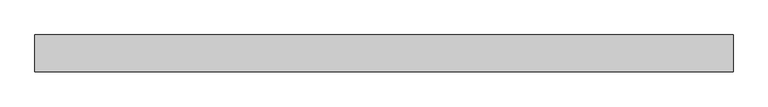
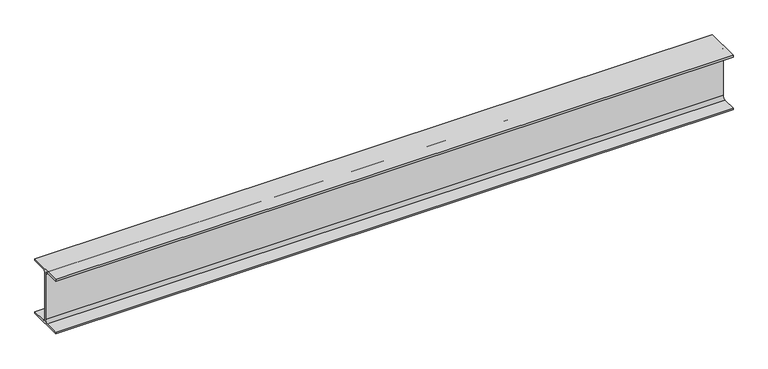
"""IFC4 building model written with IfcOpenShell, lengths in millimetres: beam geometry, 0912_Steel Framing_H-KSD3502 : H_SB_ASB_H-482x300x11x15."""

from ifc_helpers import new_model, si_unit, point, frame, frame_2d, origin, place, context, project, spatial, polyline, circle_curve, trimmed, segment, composite_curve, outline, extrude, source, transform, mapped, element, save


def beam_2ebcb970(model_context):
    return source(origin(), model_context, "Body", "SweptSolid", [
        extrude(outline(composite_curve([segment(polyline([(150.0, -226.0), (150.0, -241.0), (-150.0, -241.0), (-150.0, -226.0), (-31.5, -226.0)]), True, "CONTINUOUS"), segment(trimmed(circle_curve(frame_2d((-31.5, -200.0)), 26.0), [point((-31.5, -226.0))], [point((-5.5, -200.0))], True, "CARTESIAN"), True, "CONTINUOUS"), segment(polyline([(-5.5, -200.0), (-5.5, 200.0)]), True, "CONTINUOUS"), segment(trimmed(circle_curve(frame_2d((-31.5, 200.0)), 26.0), [point((-5.5, 200.0))], [point((-31.5, 226.0))], True, "CARTESIAN"), True, "CONTINUOUS"), segment(polyline([(-31.5, 226.0), (-150.0, 226.0), (-150.0, 241.0), (150.0, 241.0), (150.0, 226.0), (31.5, 226.0)]), True, "CONTINUOUS"), segment(trimmed(circle_curve(frame_2d((31.5, 200.0)), 26.0), [point((31.5, 226.0))], [point((5.5, 200.0))], True, "CARTESIAN"), True, "CONTINUOUS"), segment(polyline([(5.5, 200.0), (5.5, -200.0)]), True, "CONTINUOUS"), segment(trimmed(circle_curve(frame_2d((31.5, -200.0)), 26.0), [point((5.5, -200.0))], [point((31.5, -226.0))], True, "CARTESIAN"), True, "CONTINUOUS"), segment(polyline([(31.5, -226.0), (150.0, -226.0)]), True, "CONTINUOUS")], self_intersect=False)), frame((-2837.3, 0.0, 0.0), z_axis=(1.0, 0.0, 0.0), x_axis=(0.0, 1.0, 0.0)), (0.0, 0.0, 1.0), 5674.6),
    ])


if __name__ == "__main__":
    model = new_model("IFC4")
    model_context = context("Model", 3, world=origin())
    ifc_project = project(units=[si_unit("LENGTHUNIT", "METRE", prefix="MILLI")], contexts=[model_context])
    site = spatial("IfcSite", under=ifc_project)
    building = spatial("IfcBuilding", under=site)
    placement = place(None, origin())
    beam_shape = beam_2ebcb970(model_context)
    element("IfcBeam", 1, ObjectType="0912_Steel Framing_H-KSD3502 : H_SB_ASB_H-482x300x11x15", at=placement, inside=building, context=model_context, shape_type="MappedRepresentation", body=[
        mapped(beam_shape, transform((0.0, 0.0, 0.0), x_axis=(1.0, 0.0, 0.0), y_axis=(0.0, 1.0, 0.0), z_axis=(0.0, 0.0, 1.0))),
    ])
    save(model, "model.ifc")

# Revit data of these elements
# Type "0912_Steel Framing_H-KSD3502 : H_SB_ASB_H-482x300x11x15"
#   H_WM Code_1 = "S01AA001-00001 | Main Steel Structure Fabrication Work | Shelter/Building | Heavy Steel - Standard (Weight≥90KG/M) | Material: (   )"
#   H_WM Code_2 = "S03AA027-00001 | Main Steel Structure Erection Work | Shelter/Building | Heavy Steel (Weight≥90KG/M) | Material: (   )"
#   H_WM Code_3 = "S01AA010-00001 | Main Steel Structure Fabrication Work | Shelter/Building | Steel Painting/Coating | for Non-Fireproofed Steel Surface, Surface Preparation, Primer, Second & Final Coat | Material: (   )"
#   H_Q'ty Cal Type Tag = "SB-Q2"
#   Width = 30.0 cm
#   Web Thickness = 1.1 cm
#   Web Fillet = 2.6 cm
#   Warping Constant = 3680000.0 cm⁶
#   W = 0
#   Torsional Moment of Inertia = 88.2192 cm⁴
#   Section Area = 145.5 cm²
#   Plastic Modulus weak axis = 695.0 cm³
#   Plastic Modulus strong axis = 2790.0 cm³
#   Perimeter = 2.10 m²/m
#   Nominal Weight = 114.00 kgf/m
#   Moment of Inertia weak axis = 6760.00 cm⁴
#   Moment of Inertia strong axis = 60400.00 cm⁴
#   Height = 48.2 cm
#   Flange Thickness = 1.5 cm
#   Elastic Modulus weak axis = 451.0 cm³
#   Elastic Modulus strong axis = 2500.0 cm³
#   Centroid Vertical = 24.1 cm
#   Centroid Horizontal = 15.0 cm
#   Ix = 604000000
#   Length [instance default] = 1.5240 m
#   Zx = 2790000
#   b = 0.3000 m
#   h = 0.4820 m
#   r = 0.0260 m
#   s = 0.0110 m
#   t = 0.0150 m
#   A = 0.01455 m²
#   Structural Material [instance default] = Steel, 45-345
#   Assembly Code = ""
# Element 1 (IfcBeam, "0912_Steel Framing_H-KSD3502 : H_SB_ASB_H-482x300x11x15")
#   Structural Material = none
# Materials
#   "Steel, 45-345": class "Metal", colour RGB 189 187 185, transparency 0, Description = "Steel 345 MPa", Cost = 0
